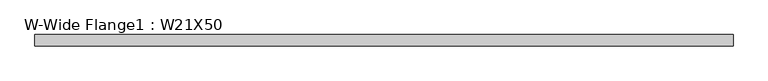
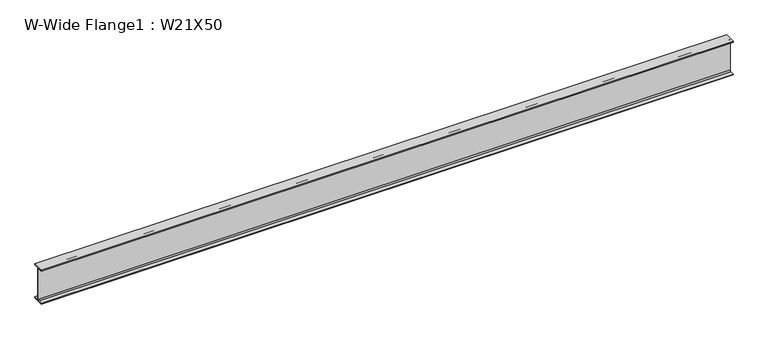
"""IFC4 building model written with IfcOpenShell, lengths in millimetres: beam geometry, W-Wide Flange1 : W21X50."""

from ifc_helpers import new_model, si_unit, point, frame, frame_2d, origin, place, context, project, spatial, polyline, circle_curve, trimmed, segment, composite_curve, outline, extrude, source, transform, mapped, element, save


def w_wide_flange1_w21x50_c6a79494(model_context):
    return source(origin(), model_context, "Body", "SweptSolid", [
        extrude(outline(composite_curve([segment(polyline([(82.931, -250.571), (82.931, -264.16), (-82.931, -264.16), (-82.931, -250.571), (-22.987, -250.571)]), True, "CONTINUOUS"), segment(trimmed(circle_curve(frame_2d((-22.987, -232.41)), 18.161), [point((-22.987, -250.571))], [point((-4.826, -232.41))], True, "CARTESIAN"), True, "CONTINUOUS"), segment(polyline([(-4.826, -232.41), (-4.826, 232.41)]), True, "CONTINUOUS"), segment(trimmed(circle_curve(frame_2d((-22.987, 232.41)), 18.161), [point((-4.826, 232.41))], [point((-22.987, 250.571))], True, "CARTESIAN"), True, "CONTINUOUS"), segment(polyline([(-22.987, 250.571), (-82.931, 250.571), (-82.931, 264.16), (82.931, 264.16), (82.931, 250.571), (22.987, 250.571)]), True, "CONTINUOUS"), segment(trimmed(circle_curve(frame_2d((22.987, 232.41)), 18.161), [point((22.987, 250.571))], [point((4.826, 232.41))], True, "CARTESIAN"), True, "CONTINUOUS"), segment(polyline([(4.826, 232.41), (4.826, -232.41)]), True, "CONTINUOUS"), segment(trimmed(circle_curve(frame_2d((22.987, -232.41)), 18.161), [point((4.826, -232.41))], [point((22.987, -250.571))], True, "CARTESIAN"), True, "CONTINUOUS"), segment(polyline([(22.987, -250.571), (82.931, -250.571)]), True, "CONTINUOUS")], self_intersect=False)), frame((-5235.0532515, 0.0, 0.0), z_axis=(1.0, 0.0, 0.0), x_axis=(0.0, 1.0, 0.0)), (0.0, 0.0, 1.0), 10267.9016134),
    ])


if __name__ == "__main__":
    model = new_model("IFC4")
    model_context = context("Model", 3, world=origin())
    ifc_project = project(units=[si_unit("LENGTHUNIT", "METRE", prefix="MILLI")], contexts=[model_context])
    site = spatial("IfcSite", under=ifc_project)
    building = spatial("IfcBuilding", under=site)
    placement = place(None, origin())
    w_wide_flange1_w21x50_shape = w_wide_flange1_w21x50_c6a79494(model_context)
    element("IfcBeam", 1, ObjectType="W-Wide Flange1 : W21X50", at=placement, inside=building, context=model_context, shape_type="MappedRepresentation", body=[
        mapped(w_wide_flange1_w21x50_shape, transform((0.0, 0.0, 0.0), x_axis=(1.0, 0.0, 0.0), y_axis=(0.0, 1.0, 0.0), z_axis=(0.0, 0.0, 1.0))),
    ])
    save(model, "model.ifc")

# Revit data of these elements
# Type "W-Wide Flange1 : W21X50"
#   Assembly Code = "B10"
#   W = 50
#   Start Extension Calculation [instance default] = 10' - 0"
#   Start Extension [instance default] = -0' - 0 1/2"
#   End Extension Calculation [instance default] = 10' - 0"
#   End Extension [instance default] = -0' - 0 1/2"
#   Length [instance default] = 5' - 0"
#   bf = 0' - 6.53"
#   d = 1' - 8.8"
#   k = 0' - 1 1/4"
#   k2 = 0' - 0.715"
#   tf = 0' - 0.535"
#   tw = 0' - 0.38"
#   A = 0.102083 SF
#   Structural Material [instance default] = Metal - Steel - ASTM A992
# Element 1 (IfcBeam, "W-Wide Flange1 : W21X50")
#   Materials on its faces: "Metal - Steel - ASTM A992"
# Materials
#   "Metal - Steel - ASTM A992": class "Metal", colour RGB 199 199 199, transparency 0
